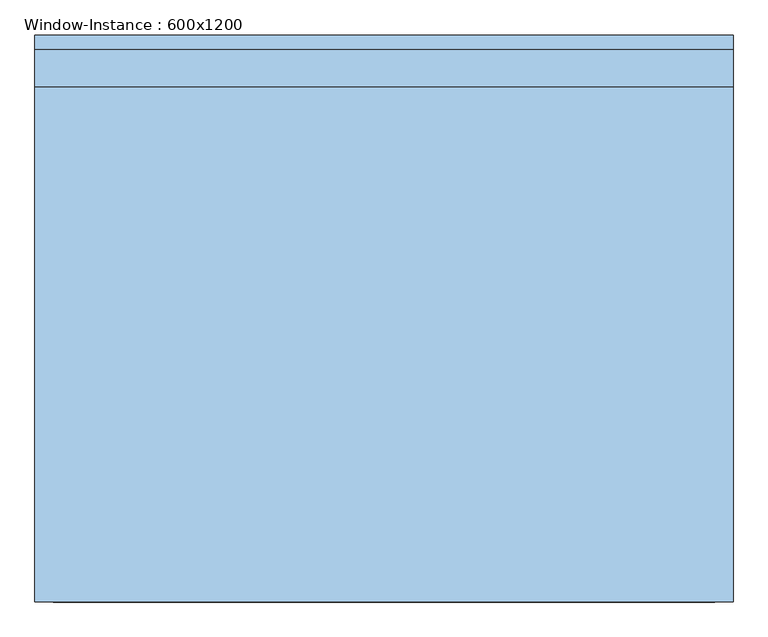
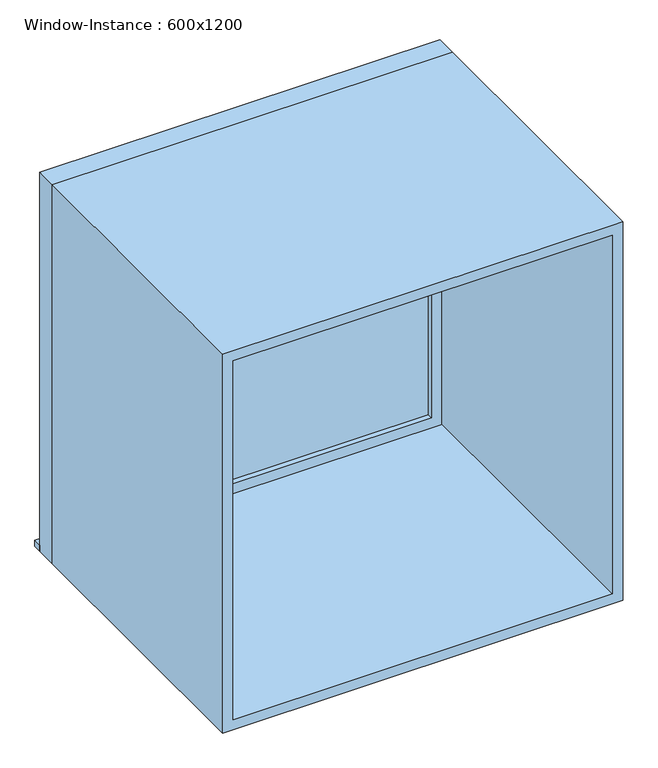
"""IFC4 building model written with IfcOpenShell, lengths in millimetres: window geometry, Window-Instance : 600x1200."""

from ifc_helpers import new_model, si_unit, frame, origin, place, context, project, spatial, polyline, outline, extrude, source, transform, mapped, element, save


def window_instance_600x1200_bc87a244(model_context):
    return source(origin(), model_context, "Body", "SweptSolid", [
        extrude(outline(polyline([(-638.1, 500.4), (561.9, 500.4), (561.9, 475.0), (-638.1, 475.0), (-638.1, 500.4)])), frame((0.0, 0.0, 900.0), z_axis=(0.0, 0.0, 1.0), x_axis=(1.0, 0.0, 0.0)), (0.0, 0.0, 1.0), 19.05),
        extrude(outline(polyline([(498.4, 426.425), (-574.6, 426.425), (-574.6, 439.125), (498.4, 439.125), (498.4, 426.425)])), frame((0.0, 0.0, 963.5), z_axis=(0.0, 0.0, 1.0), x_axis=(1.0, 0.0, 0.0)), (0.0, 0.0, 1.0), 1073.0),
        extrude(outline(polyline([(2080.95, -619.05), (919.05, -619.05), (919.05, 542.85), (2080.95, 542.85), (2080.95, -619.05)]), holes=[polyline([(2036.5, -574.6), (2036.5, 498.4), (963.5, 498.4), (963.5, -574.6), (2036.5, -574.6)])]), frame((0.0, 410.55, 0.0), z_axis=(0.0, 1.0, 0.0), x_axis=(0.0, 0.0, 1.0)), (0.0, 0.0, 1.0), 44.45),
        extrude(outline(polyline([(2100.0, -638.1), (900.0, -638.1), (900.0, 561.9), (2100.0, 561.9), (2100.0, -638.1)]), holes=[polyline([(2068.25, -606.35), (2068.25, 530.15), (931.75, 530.15), (931.75, -606.35), (2068.25, -606.35)])]), frame((0.0, -475.0, 0.0), z_axis=(0.0, 1.0, 0.0), x_axis=(0.0, 0.0, 1.0)), (0.0, 0.0, 1.0), 885.55),
        extrude(outline(polyline([(2100.0, 561.9), (2100.0, -638.1), (900.0, -638.1), (900.0, 561.9), (2100.0, 561.9)]), holes=[polyline([(2080.95, 542.85), (919.05, 542.85), (919.05, -619.05), (2080.95, -619.05), (2080.95, 542.85)])]), frame((0.0, 410.55, 0.0), z_axis=(0.0, 1.0, 0.0), x_axis=(0.0, 0.0, 1.0)), (0.0, 0.0, 1.0), 64.45),
    ])


if __name__ == "__main__":
    model = new_model("IFC4")
    model_context = context("Model", 3, world=origin())
    ifc_project = project(units=[si_unit("LENGTHUNIT", "METRE", prefix="MILLI")], contexts=[model_context])
    site = spatial("IfcSite", under=ifc_project)
    building = spatial("IfcBuilding", under=site)
    placement = place(None, origin())
    window_instance_600x1200_shape = window_instance_600x1200_bc87a244(model_context)
    element("IfcWindow", 1, ObjectType="Window-Instance : 600x1200", at=placement, inside=building, context=model_context, shape_type="MappedRepresentation", body=[
        mapped(window_instance_600x1200_shape, transform((0.0, 0.0, 0.0), x_axis=(1.0, 0.0, 0.0), y_axis=(0.0, 1.0, 0.0), z_axis=(0.0, 0.0, 1.0))),
    ])
    save(model, "model.ifc")

# Revit data of these elements
# Type "Window-Instance : 600x1200"
#   Type Mark = "7"
#   Construction Type Id = "GSP4R"
#   Assembly Code = "B2020100"
#   Analytic Construction = "1/8 in Pilkington single glazing"
#   Visual Light Transmittance = 0.9
#   Thermal Resistance (R) = 0.149095 (m²·K)/W
#   Solar Heat Gain Coefficient = 0.86
#   Heat Transfer Coefficient (U) = 6.70716 W/(m²·K)
#   Height [instance default] = 1200 mm
#   Default Sill Height = 900 mm
#   Width [instance default] = 600 mm
#   Window Inset = 20 mm
#   Glass Pane Material = WW-EC-GL-Storefront
#   Sash Material = WW-EC-RGB-White
#   Wall Closure = (empty or 0)
# Element 1 (IfcWindow, "Window-Instance : 600x1200")
#   Width = 1200 mm
#   Materials on its faces: "WW-EC-RGB-White", "WW-EC-GL-Storefront"
# Materials
#   "WW-EC-GL-Storefront": class "Glass", colour RGB 236 240 239, transparency 0.85, Description = "Storefront Glass", Cost = 0
#   "WW-EC-RGB-White": class "Generic", colour RGB 255 255 255, transparency 0, Comments = "If region requests off-white, swith asset color to RGB 231-228-220", Description = "Generic Color", Cost = 0
